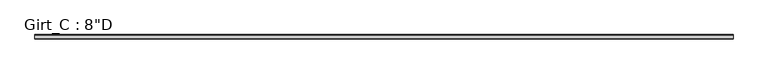
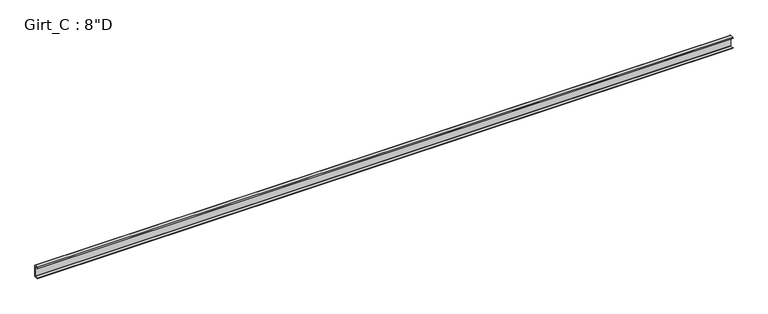
"""IFC4 building model written with IfcOpenShell, lengths in millimetres: beam geometry."""

from ifc_helpers import new_model, si_unit, point, frame, frame_2d, origin, place, context, project, spatial, polyline, circle_curve, trimmed, segment, composite_curve, outline, extrude, source, transform, mapped, element, save


def beam_06ba003b(model_context):
    return source(origin(), model_context, "Body", "SweptSolid", [
        extrude(outline(composite_curve([segment(polyline([(-63.5, 101.6), (-3.3734375, 101.6)]), True, "CONTINUOUS"), segment(trimmed(circle_curve(frame_2d((-3.3734375, 96.8375)), 4.7625), [point((-3.3734375, 101.6))], [point((1.3890625, 96.8375))], False, "CARTESIAN"), True, "CONTINUOUS"), segment(polyline([(1.3890625, 96.8375), (1.3890625, -96.8375)]), True, "CONTINUOUS"), segment(trimmed(circle_curve(frame_2d((-3.3734375, -96.8375)), 4.7625), [point((1.3890625, -96.8375))], [point((-3.3734375, -101.6))], False, "CARTESIAN"), True, "CONTINUOUS"), segment(polyline([(-3.3734375, -101.6), (-63.5, -101.6), (-75.745104, -87.0068534), (-73.6169367, -85.221109), (-62.204539, -98.821875), (-3.2694106, -98.821875)]), True, "CONTINUOUS"), segment(trimmed(circle_curve(frame_2d((-3.3748024, -96.8389339)), 1.9857399), [point((-3.2694106, -98.821875))], [point((-1.3890625, -96.8389339))], True, "CARTESIAN"), True, "CONTINUOUS"), segment(polyline([(-1.3890625, -96.8389339), (-1.3890625, 96.8381931)]), True, "CONTINUOUS"), segment(trimmed(circle_curve(frame_2d((-3.3741066, 96.8381931)), 1.9850441), [point((-1.3890625, 96.8381931))], [point((-3.3005807, 98.821875))], True, "CARTESIAN"), True, "CONTINUOUS"), segment(polyline([(-3.3005807, 98.821875), (-62.204539, 98.821875), (-73.6169367, 85.221109), (-75.745104, 87.0068534), (-63.5, 101.6)]), True, "CONTINUOUS")], self_intersect=False)), frame((-5979.31875, 0.0, 0.0), z_axis=(1.0, 0.0, 0.0), x_axis=(0.0, 1.0, 0.0)), (0.0, 0.0, 1.0), 11958.6375),
    ])


if __name__ == "__main__":
    model = new_model("IFC4")
    model_context = context("Model", 3, world=origin())
    ifc_project = project(units=[si_unit("LENGTHUNIT", "METRE", prefix="MILLI")], contexts=[model_context])
    site = spatial("IfcSite", under=ifc_project)
    building = spatial("IfcBuilding", under=site)
    placement = place(None, origin())
    beam_shape = beam_06ba003b(model_context)
    element("IfcBeam", 1, ObjectType="Girt_C : 8\"D", at=placement, inside=building, context=model_context, shape_type="MappedRepresentation", body=[
        mapped(beam_shape, transform((0.0, 0.0, 0.0), x_axis=(1.0, 0.0, 0.0), y_axis=(0.0, 1.0, 0.0), z_axis=(0.0, 0.0, 1.0))),
    ])
    save(model, "model.ifc")

# Revit data of these elements
# Type "Girt_C : 8\"D"
#   Web_Thickness = 0' - 0 7/64"
#   Length [instance default] = 10' - 0"
#   Leg_1 = 0' - 2 1/2"
#   Height = 0' - 8"
#   Structural Material [instance default] = none
# Element 1 (IfcBeam, "Girt_C : 8\"D")
#   Structural Material = Steel
#   Materials on its faces: "Steel"
# Materials
#   "Steel": class "Metal", colour RGB 118 118 114, transparency 0, Description = "Steel, mill finish", Cost = 0
